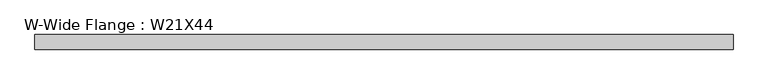
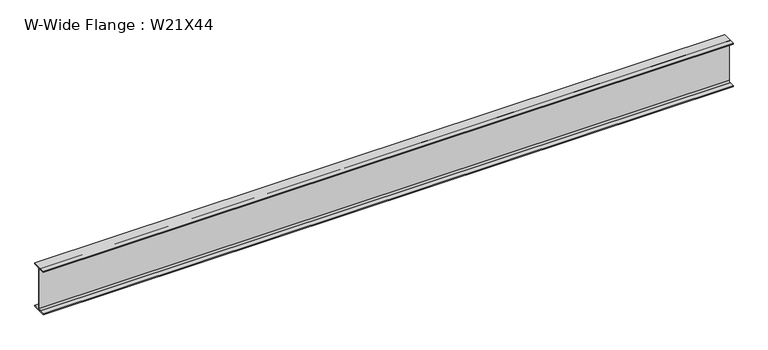
"""IFC4 building model written with IfcOpenShell, lengths in millimetres: beam geometry, W-Wide Flange : W21X44."""

from ifc_helpers import new_model, si_unit, point, frame, frame_2d, origin, place, context, project, spatial, polyline, circle_curve, trimmed, segment, composite_curve, outline, extrude, source, transform, mapped, element, save


def w_wide_flange_w21x44_aedf4de2(model_context):
    return source(origin(), model_context, "Body", "SweptSolid", [
        extrude(outline(composite_curve([segment(polyline([(82.55, -251.46), (82.55, -262.89), (-82.55, -262.89), (-82.55, -251.46), (-21.59, -251.46)]), True, "CONTINUOUS"), segment(trimmed(circle_curve(frame_2d((-21.59, -234.315)), 17.145), [point((-21.59, -251.46))], [point((-4.445, -234.315))], True, "CARTESIAN"), True, "CONTINUOUS"), segment(polyline([(-4.445, -234.315), (-4.445, 234.315)]), True, "CONTINUOUS"), segment(trimmed(circle_curve(frame_2d((-21.59, 234.315)), 17.145), [point((-4.445, 234.315))], [point((-21.59, 251.46))], True, "CARTESIAN"), True, "CONTINUOUS"), segment(polyline([(-21.59, 251.46), (-82.55, 251.46), (-82.55, 262.89), (82.55, 262.89), (82.55, 251.46), (21.59, 251.46)]), True, "CONTINUOUS"), segment(trimmed(circle_curve(frame_2d((21.59, 234.315)), 17.145), [point((21.59, 251.46))], [point((4.445, 234.315))], True, "CARTESIAN"), True, "CONTINUOUS"), segment(polyline([(4.445, 234.315), (4.445, -234.315)]), True, "CONTINUOUS"), segment(trimmed(circle_curve(frame_2d((21.59, -234.315)), 17.145), [point((4.445, -234.315))], [point((21.59, -251.46))], True, "CARTESIAN"), True, "CONTINUOUS"), segment(polyline([(21.59, -251.46), (82.55, -251.46)]), True, "CONTINUOUS")], self_intersect=False)), frame((-3907.705568, 0.0, 0.0), z_axis=(1.0, 0.0, 0.0), x_axis=(0.0, 1.0, 0.0)), (0.0, 0.0, 1.0), 7875.9910422),
    ])


if __name__ == "__main__":
    model = new_model("IFC4")
    model_context = context("Model", 3, world=origin())
    ifc_project = project(units=[si_unit("LENGTHUNIT", "METRE", prefix="MILLI")], contexts=[model_context])
    site = spatial("IfcSite", under=ifc_project)
    building = spatial("IfcBuilding", under=site)
    placement = place(None, origin())
    w_wide_flange_w21x44_shape = w_wide_flange_w21x44_aedf4de2(model_context)
    element("IfcBeam", 1, ObjectType="W-Wide Flange : W21X44", at=placement, inside=building, context=model_context, shape_type="MappedRepresentation", body=[
        mapped(w_wide_flange_w21x44_shape, transform((0.0, 0.0, 0.0), x_axis=(1.0, 0.0, 0.0), y_axis=(0.0, 1.0, 0.0), z_axis=(0.0, 0.0, 1.0))),
    ])
    save(model, "model.ifc")

# Revit data of these elements
# Type "W-Wide Flange : W21X44"
#   Assembly Code = "B10"
#   W = 44
#   Length [instance default] = 1524 mm
#   bf = 165.1 mm
#   d = 525.78 mm
#   k = 28.575 mm
#   k2 = 17.145 mm
#   tf = 11.43 mm
#   tw = 8.89 mm
#   A = 0.00838708 m²
#   Structural Material [instance default] = Steel ASTM A992
# Element 1 (IfcBeam, "W-Wide Flange : W21X44")
#   Structural Material = Aluminum, Anodized Red
#   Materials on its faces: "Aluminum, Anodized Red"
# Materials
#   "Steel ASTM A992": class "Metal", colour RGB 128 0 0, transparency 0, Description = "Structural steel 50ksi", Cost = 0
#   "Aluminum, Anodized Red": class "Metal", colour RGB 120 120 120, transparency 0, Description = "Anodized aluminum, red", Cost = 0
